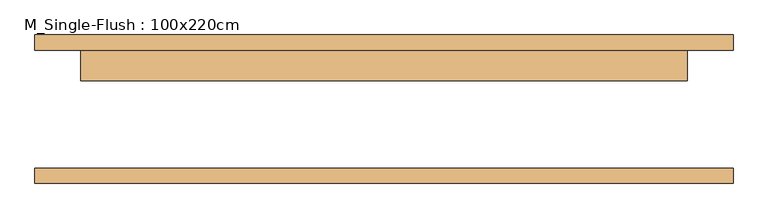
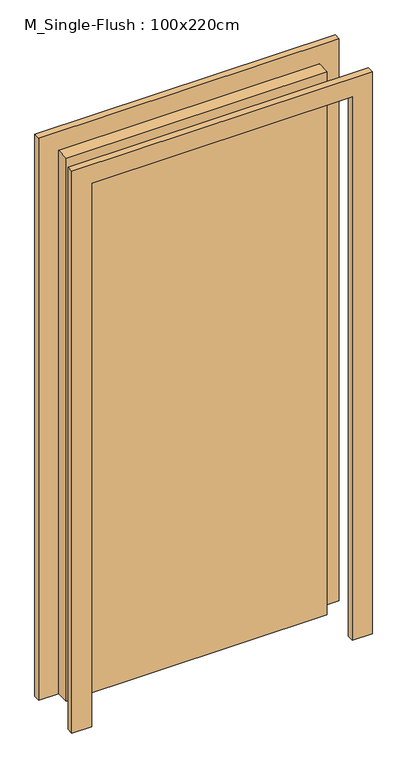
"""IFC4 building model written with IfcOpenShell, lengths in millimetres: door geometry, M_Single-Flush : 100x220cm."""

from ifc_helpers import new_model, si_unit, frame, origin, origin_with_axes, place, context, project, spatial, polyline, outline, extrude, source, transform, mapped, element, save


def m_single_flush_100x220cm_537bd306(model_context):
    return source(origin(), model_context, "Body", "SweptSolid", [
        extrude(outline(polyline([(2276.0, -576.0), (0.0, -576.0), (0.0, -500.0), (2200.0, -500.0), (2200.0, 500.0), (0.0, 500.0), (0.0, 576.0), (2276.0, 576.0), (2276.0, -576.0)])), frame((0.0, 97.5, 0.0), z_axis=(0.0, 1.0, 0.0), x_axis=(0.0, 0.0, 1.0)), (0.0, 0.0, 1.0), 25.0),
        extrude(outline(polyline([(2276.0, 576.0), (2276.0, -576.0), (0.0, -576.0), (0.0, -500.0), (2200.0, -500.0), (2200.0, 500.0), (0.0, 500.0), (0.0, 576.0), (2276.0, 576.0)])), frame((0.0, -122.5, 0.0), z_axis=(0.0, 1.0, 0.0), x_axis=(0.0, 0.0, 1.0)), (0.0, 0.0, 1.0), 25.0),
        extrude(outline(polyline([(500.0, 46.5), (-500.0, 46.5), (-500.0, 97.5), (500.0, 97.5), (500.0, 46.5)])), origin_with_axes(), (0.0, 0.0, 1.0), 2200.0),
    ])


if __name__ == "__main__":
    model = new_model("IFC4")
    model_context = context("Model", 3, world=origin())
    ifc_project = project(units=[si_unit("LENGTHUNIT", "METRE", prefix="MILLI")], contexts=[model_context])
    site = spatial("IfcSite", under=ifc_project)
    building = spatial("IfcBuilding", under=site)
    placement = place(None, origin())
    m_single_flush_100x220cm_shape = m_single_flush_100x220cm_537bd306(model_context)
    element("IfcDoor", 1, ObjectType="M_Single-Flush : 100x220cm", at=placement, inside=building, context=model_context, shape_type="MappedRepresentation", body=[
        mapped(m_single_flush_100x220cm_shape, transform((0.0, 0.0, 0.0), x_axis=(1.0, 0.0, 0.0), y_axis=(0.0, 1.0, 0.0), z_axis=(0.0, 0.0, 1.0))),
    ])
    save(model, "model.ifc")

# Revit data of these elements
# Type "M_Single-Flush : 100x220cm"
#   Type Mark = "44"
#   Construction Type Id = "MDOOR"
#   Analytic Construction = "Metal"
#   Thickness = 5.10 cm
#   Heat Transfer Coefficient (U) = 3.7021 W/(m²·K)
#   Height = 220.00 cm
#   Trim Projection Ext = 2.50 cm
#   Trim Projection Int = 2.50 cm
#   Trim Width = 7.60 cm
#   Width = 100.00 cm
#   Define Thermal Properties by = 1
#   Door Material = Door - Panel
#   Frame Material = Door - Frame
#   Visual Light Transmittance = 0
#   Solar Heat Gain Coefficient = 0
#   Function = (empty or 0)
#   Wall Closure = (empty or 0)
# Element 1 (IfcDoor, "M_Single-Flush : 100x220cm")
#   Materials on its faces: "Door - Frame", "Door - Panel"
# Materials
#   "Door - Panel": class "Wood", colour RGB 210 159 95, transparency 0, Cost = 0
#   "Door - Frame": class "Miscellaneous", colour RGB 118 70 51, transparency 0, Cost = 0
